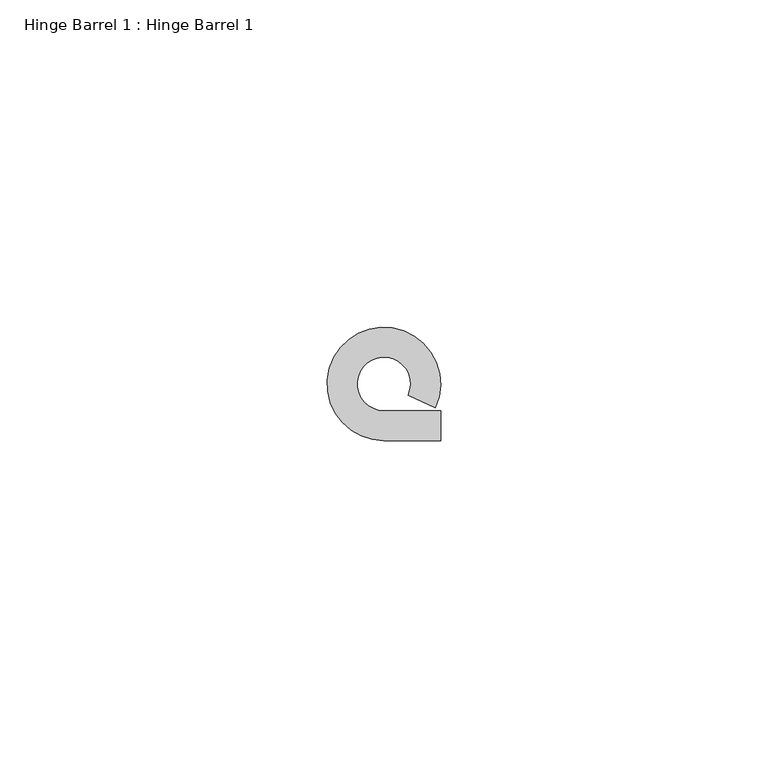
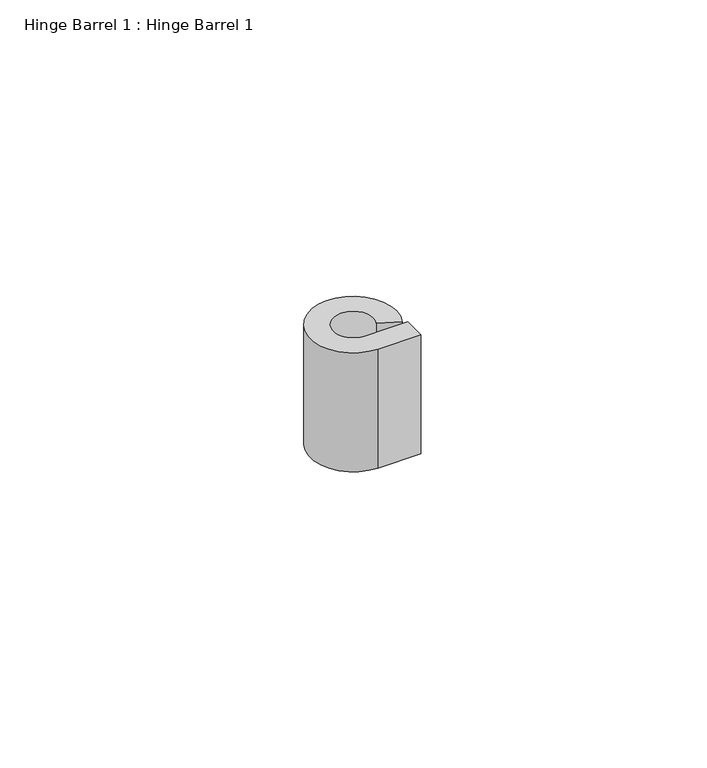
"""IFC4 building model written with IfcOpenShell, lengths in millimetres: proxy geometry, Hinge Barrel 1 : Hinge Barrel 1."""

from ifc_helpers import new_model, si_unit, point, frame, frame_2d, origin, place, context, project, spatial, polyline, circle_curve, trimmed, segment, composite_curve, outline, extrude, source, transform, mapped, element, save


def hinge_barrel_1_hinge_barrel_1_117a87e6(model_context):
    return source(origin(), model_context, "Body", "SweptSolid", [
        extrude(outline(composite_curve([segment(polyline([(587323.2214739, -531780.6943841), (587327.7934739, -531780.6943841), (587327.7934739, -531785.2584466), (587319.1320739, -531785.2584466)]), True, "CONTINUOUS"), segment(trimmed(circle_curve(frame_2d((587319.1320739, -531776.6049841)), 8.6534625), [point((587319.1320739, -531785.2584466))], [point((587326.986084, -531780.2377433))], False, "CARTESIAN"), True, "CONTINUOUS"), segment(polyline([(587326.986084, -531780.2377433), (587322.8436736, -531778.321731)]), True, "CONTINUOUS"), segment(trimmed(circle_curve(frame_2d((587319.1320739, -531776.6049841)), 4.0894), [point((587322.8436736, -531778.321731))], [point((587319.1320739, -531780.6943841))], True, "CARTESIAN"), True, "CONTINUOUS"), segment(polyline([(587319.1320739, -531780.6943841), (587323.2214739, -531780.6943841)]), True, "CONTINUOUS")], self_intersect=False)), frame((0.0, 0.0, 311.15), z_axis=(0.0, 0.0, 1.0), x_axis=(1.0, 0.0, 0.0)), (0.0, 0.0, 1.0), 25.4),
    ])


if __name__ == "__main__":
    model = new_model("IFC4")
    model_context = context("Model", 3, world=origin())
    ifc_project = project(units=[si_unit("LENGTHUNIT", "METRE", prefix="MILLI")], contexts=[model_context])
    site = spatial("IfcSite", under=ifc_project)
    building = spatial("IfcBuilding", under=site)
    placement = place(None, origin())
    hinge_barrel_1_hinge_barrel_1_shape = hinge_barrel_1_hinge_barrel_1_117a87e6(model_context)
    element("IfcBuildingElementProxy", 1, Name="Hinge Barrel 1 : Hinge Barrel 1", ObjectType="Hinge Barrel 1 : Hinge Barrel 1", at=placement, inside=building, context=model_context, shape_type="MappedRepresentation", body=[
        mapped(hinge_barrel_1_hinge_barrel_1_shape, transform((0.0, 0.0, 0.0), x_axis=(1.0, 0.0, 0.0), y_axis=(0.0, 1.0, 0.0), z_axis=(0.0, 0.0, 1.0))),
    ])
    save(model, "model.ifc")

# Revit data of these elements
# Element 1 (IfcBuildingElementProxy, "Hinge Barrel 1 : Hinge Barrel 1")
#   Materials on its faces: "6\"X6\" WELD-ON STL BUTT HINGE"
# Materials
#   "6\"X6\" WELD-ON STL BUTT HINGE": class "Metal", colour RGB 189 187 185, transparency 0, Description = "Carbon steel", Cost = 0
